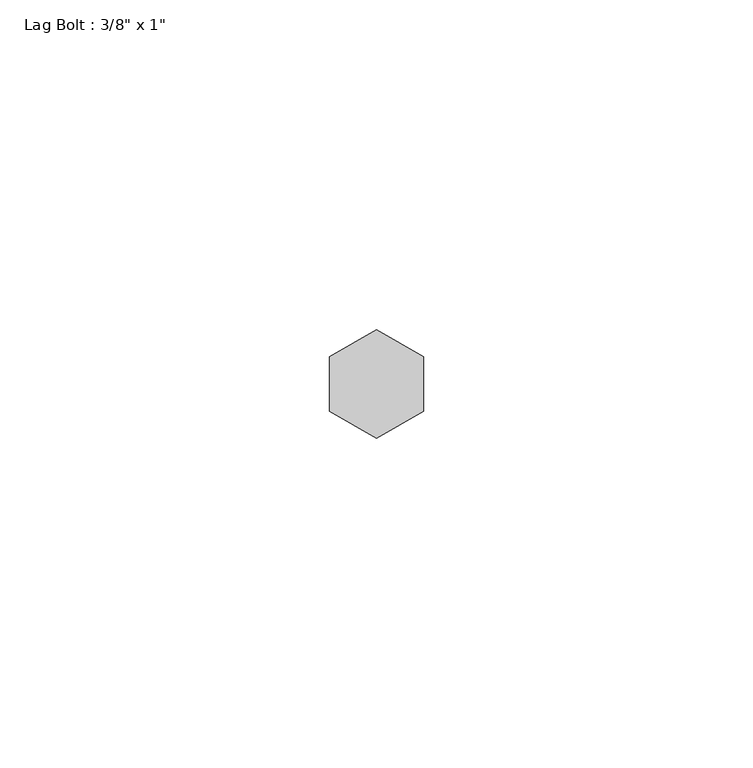
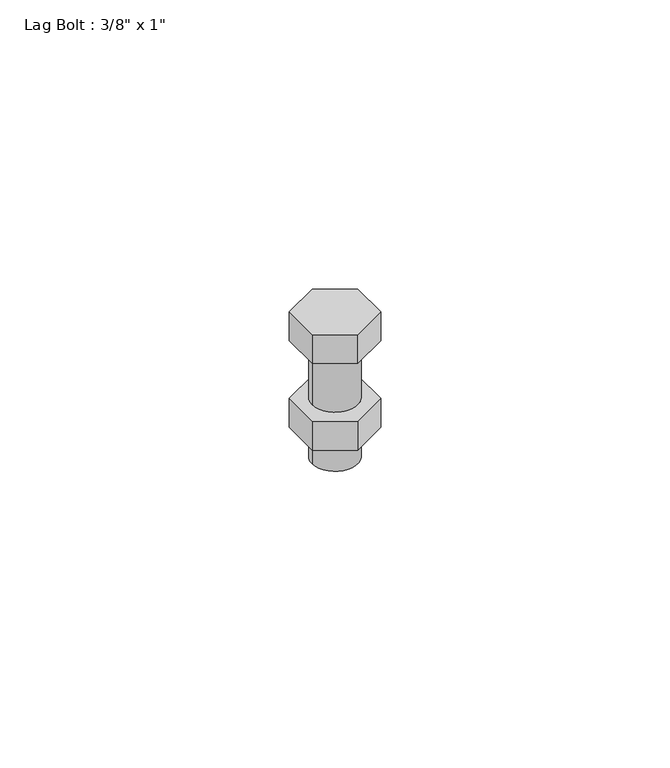
"""IFC4 building model written with IfcOpenShell, lengths in millimetres: proxy geometry."""

from ifc_helpers import new_model, si_unit, point, frame, origin, origin_with_axes, origin_2d, place, context, project, spatial, polyline, circle_curve, trimmed, segment, composite_curve, outline, extrude, source, transform, mapped, element, save


def proxy_bc53a808(model_context):
    return source(origin(), model_context, "Body", "SweptSolid", [
        extrude(outline(polyline([(-7.14375, 4.124446), (0.0, 8.248892), (7.14375, 4.124446), (7.14375, -4.124446), (0.0, -8.248892), (-7.14375, -4.124446), (-7.14375, 4.124446)])), frame((0.0, 0.0, -19.05), z_axis=(0.0, 0.0, 1.0), x_axis=(1.0, 0.0, 0.0)), (0.0, 0.0, 1.0), 6.35),
        extrude(outline(polyline([(-7.14375, -4.124446), (-7.14375, 4.124446), (0.0, 8.248892), (7.14375, 4.124446), (7.14375, -4.124446), (0.0, -8.248892), (-7.14375, -4.124446)])), origin_with_axes(), (0.0, 0.0, 1.0), 6.35),
        extrude(outline(composite_curve([segment(trimmed(circle_curve(origin_2d(), 4.7625), [point((-4.7625, 0.0))], [point((4.7625, 0.0))], False, "CARTESIAN"), True, "CONTINUOUS"), segment(trimmed(circle_curve(origin_2d(), 4.7625), [point((4.7625, 0.0))], [point((-4.7625, 0.0))], False, "CARTESIAN"), True, "CONTINUOUS")], self_intersect=False)), frame((0.0, 0.0, -25.4), z_axis=(0.0, 0.0, 1.0), x_axis=(1.0, 0.0, 0.0)), (0.0, 0.0, 1.0), 25.4),
    ])


if __name__ == "__main__":
    model = new_model("IFC4")
    model_context = context("Model", 3, world=origin())
    ifc_project = project(units=[si_unit("LENGTHUNIT", "METRE", prefix="MILLI")], contexts=[model_context])
    site = spatial("IfcSite", under=ifc_project)
    building = spatial("IfcBuilding", under=site)
    placement = place(None, origin())
    proxy_shape = proxy_bc53a808(model_context)
    element("IfcBuildingElementProxy", 1, Name="Lag Bolt : 3/8\" x 1\"", ObjectType="Lag Bolt : 3/8\" x 1\"", at=placement, inside=building, context=model_context, shape_type="MappedRepresentation", body=[
        mapped(proxy_shape, transform((0.0, 0.0, 0.0), x_axis=(1.0, 0.0, 0.0), y_axis=(0.0, 1.0, 0.0), z_axis=(0.0, 0.0, 1.0))),
    ])
    save(model, "model.ifc")

# Revit data of these elements
# Type "Lag Bolt : 3/8\" x 1\""
#   Thickness_of_Substrate [instance default] = 0' - 1"
#   Side = 0' - 0.3252"
#   Radius = 0' - 0 3/16"
#   Length = 0' - 1"
#   Head Size = 0' - 0 9/16"
#   Head Radius = 0' - 0 9/32"
#   Head Height = 0' - 0 1/4"
#   Diameter = 0' - 0 3/8"
#   Default Elevation = 4' - 0"
#   Nut_Visibility [instance default] = yes
#   Bolt Material (Size) [instance default] = STRUCTURAL BOLTS (PAINT TO MATCH STEEL FINISH)
# Element 1 (IfcBuildingElementProxy, "Lag Bolt : 3/8\" x 1\"")
#   Thickness_of_Substrate = 0' - 0 1/2"
#   Bolt Material (Size) = 3/8" X 1" GALV. BOLTS
#   Materials on its faces: "3/8\" X 1\" GALV. BOLTS", "STRUCTURAL BOLTS (PAINT TO MATCH STEEL FINISH)"
# Materials
#   "STRUCTURAL BOLTS (PAINT TO MATCH STEEL FINISH)": class "Generic", colour RGB 120 120 120, transparency 0, Cost = 0
#   "3/8\" X 1\" GALV. BOLTS": class "Generic", colour RGB 120 120 120, transparency 0, Cost = 0
